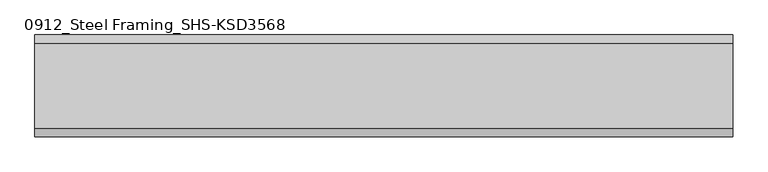
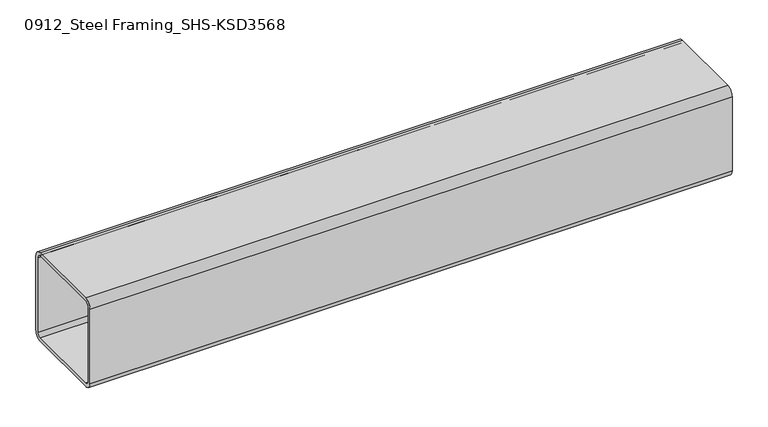
"""IFC4 building model written with IfcOpenShell, lengths in millimetres: beam geometry, 0912_Steel Framing_SHS-KSD3568 : H_SB_ASB_SHS-150x150x6."""

from ifc_helpers import new_model, si_unit, point, frame, frame_2d, origin, place, context, project, spatial, polyline, circle_curve, trimmed, segment, composite_curve, outline, extrude, source, transform, mapped, element, save


def beam_0912_steel_framing_shs_ksd3568_83a256cf(model_context):
    return source(origin(), model_context, "Body", "SweptSolid", [
        extrude(outline(composite_curve([segment(polyline([(75.0, 63.0), (75.0, -63.0)]), True, "CONTINUOUS"), segment(trimmed(circle_curve(frame_2d((63.0, -63.0)), 12.0), [point((75.0, -63.0))], [point((63.0, -75.0))], False, "CARTESIAN"), True, "CONTINUOUS"), segment(polyline([(63.0, -75.0), (-63.0, -75.0)]), True, "CONTINUOUS"), segment(trimmed(circle_curve(frame_2d((-63.0, -63.0)), 12.0), [point((-63.0, -75.0))], [point((-75.0, -63.0))], False, "CARTESIAN"), True, "CONTINUOUS"), segment(polyline([(-75.0, -63.0), (-75.0, 63.0)]), True, "CONTINUOUS"), segment(trimmed(circle_curve(frame_2d((-63.0, 63.0)), 12.0), [point((-75.0, 63.0))], [point((-63.0, 75.0))], False, "CARTESIAN"), True, "CONTINUOUS"), segment(polyline([(-63.0, 75.0), (63.0, 75.0)]), True, "CONTINUOUS"), segment(trimmed(circle_curve(frame_2d((63.0, 63.0)), 12.0), [point((63.0, 75.0))], [point((75.0, 63.0))], False, "CARTESIAN"), True, "CONTINUOUS")], self_intersect=False), holes=[composite_curve([segment(trimmed(circle_curve(frame_2d((-63.0, 63.0)), 6.0), [point((-63.0, 69.0))], [point((-69.0, 63.0))], True, "CARTESIAN"), True, "CONTINUOUS"), segment(polyline([(-69.0, 63.0), (-69.0, -63.0)]), True, "CONTINUOUS"), segment(trimmed(circle_curve(frame_2d((-63.0, -63.0)), 6.0), [point((-69.0, -63.0))], [point((-63.0, -69.0))], True, "CARTESIAN"), True, "CONTINUOUS"), segment(polyline([(-63.0, -69.0), (63.0, -69.0)]), True, "CONTINUOUS"), segment(trimmed(circle_curve(frame_2d((63.0, -63.0)), 6.0), [point((63.0, -69.0))], [point((69.0, -63.0))], True, "CARTESIAN"), True, "CONTINUOUS"), segment(polyline([(69.0, -63.0), (69.0, 63.0)]), True, "CONTINUOUS"), segment(trimmed(circle_curve(frame_2d((63.0, 63.0)), 6.0), [point((69.0, 63.0))], [point((63.0, 69.0))], True, "CARTESIAN"), True, "CONTINUOUS"), segment(polyline([(63.0, 69.0), (-63.0, 69.0)]), True, "CONTINUOUS")], self_intersect=False)]), frame((-515.0, 0.0, 0.0), z_axis=(1.0, 0.0, 0.0), x_axis=(0.0, 1.0, 0.0)), (0.0, 0.0, 1.0), 1030.0),
    ])


if __name__ == "__main__":
    model = new_model("IFC4")
    model_context = context("Model", 3, world=origin())
    ifc_project = project(units=[si_unit("LENGTHUNIT", "METRE", prefix="MILLI")], contexts=[model_context])
    site = spatial("IfcSite", under=ifc_project)
    building = spatial("IfcBuilding", under=site)
    placement = place(None, origin())
    beam_0912_steel_framing_shs_ksd3568_shape = beam_0912_steel_framing_shs_ksd3568_83a256cf(model_context)
    element("IfcBeam", 1, ObjectType="0912_Steel Framing_SHS-KSD3568 : H_SB_ASB_SHS-150x150x6", at=placement, inside=building, context=model_context, shape_type="MappedRepresentation", body=[
        mapped(beam_0912_steel_framing_shs_ksd3568_shape, transform((0.0, 0.0, 0.0), x_axis=(1.0, 0.0, 0.0), y_axis=(0.0, 1.0, 0.0), z_axis=(0.0, 0.0, 1.0))),
    ])
    save(model, "model.ifc")

# Revit data of these elements
# Type "0912_Steel Framing_SHS-KSD3568 : H_SB_ASB_SHS-150x150x6"
#   H_WM Code_1 = "S01AA002-00001 | Main Steel Structure Fabrication Work | Shelter/Building | Medium Steel - Standard (90KG/M>Weight≥30KG/M) | Material: (   )"
#   H_WM Code_2 = "S03AA028-00001 | Main Steel Structure Erection Work | Shelter/Building | Medium Steel (90KG/M>Weight≥30KG/M) | Material: (   )"
#   H_WM Code_3 = "S01AA010-00001 | Main Steel Structure Fabrication Work | Shelter/Building | Steel Painting/Coating | for Non-Fireproofed Steel Surface, Surface Preparation, Primer, Second & Final Coat | Material: (   )"
#   H_Q'ty Cal Type Tag = "SB-Q2"
#   Perimeter = 0.60 m²/m
#   Nominal Weight = 26.40 kgf/m
#   Length [instance default] = 1.0000 m
#   b = 0.1500 m
#   h = 0.1500 m
#   tr = 0.0120 m
#   t = 0.0060 m
#   A = 28.36 m²
#   Structural Material [instance default] = Steel, 45-345
# Element 1 (IfcBeam, "0912_Steel Framing_SHS-KSD3568 : H_SB_ASB_SHS-150x150x6")
#   Structural Material = none
# Materials
#   "Steel, 45-345": class "Metal", colour RGB 189 187 185, transparency 0, Description = "Steel 345 MPa", Cost = 0
